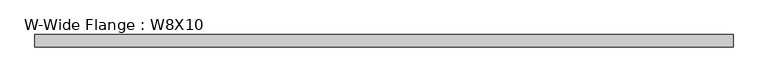
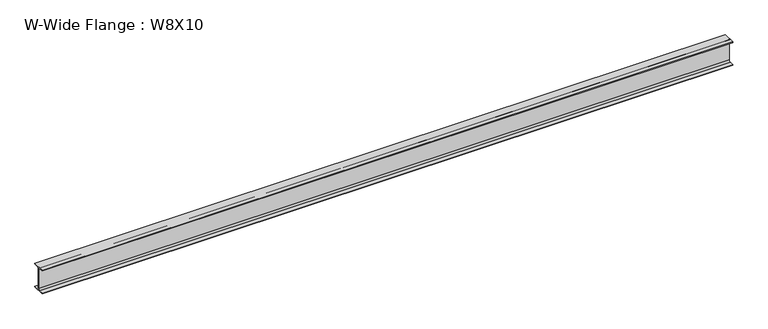
"""IFC4 building model written with IfcOpenShell, lengths in millimetres: beam geometry, W-Wide Flange : W8X10."""

from ifc_helpers import new_model, si_unit, point, frame, frame_2d, origin, place, context, project, spatial, polyline, circle_curve, trimmed, segment, composite_curve, outline, extrude, source, transform, mapped, element, save


def w_wide_flange_w8x10_6a41b71d(model_context):
    return source(origin(), model_context, "Body", "SweptSolid", [
        extrude(outline(composite_curve([segment(polyline([(50.038, -94.996), (50.038, -100.203), (-50.038, -100.203), (-50.038, -94.996), (-14.4145, -94.996)]), True, "CONTINUOUS"), segment(trimmed(circle_curve(frame_2d((-14.4145, -82.7405)), 12.2555), [point((-14.4145, -94.996))], [point((-2.159, -82.7405))], True, "CARTESIAN"), True, "CONTINUOUS"), segment(polyline([(-2.159, -82.7405), (-2.159, 82.7405)]), True, "CONTINUOUS"), segment(trimmed(circle_curve(frame_2d((-14.4145, 82.7405)), 12.2555), [point((-2.159, 82.7405))], [point((-14.4145, 94.996))], True, "CARTESIAN"), True, "CONTINUOUS"), segment(polyline([(-14.4145, 94.996), (-50.038, 94.996), (-50.038, 100.203), (50.038, 100.203), (50.038, 94.996), (14.4145, 94.996)]), True, "CONTINUOUS"), segment(trimmed(circle_curve(frame_2d((14.4145, 82.7405)), 12.2555), [point((14.4145, 94.996))], [point((2.159, 82.7405))], True, "CARTESIAN"), True, "CONTINUOUS"), segment(polyline([(2.159, 82.7405), (2.159, -82.7405)]), True, "CONTINUOUS"), segment(trimmed(circle_curve(frame_2d((14.4145, -82.7405)), 12.2555), [point((2.159, -82.7405))], [point((14.4145, -94.996))], True, "CARTESIAN"), True, "CONTINUOUS"), segment(polyline([(14.4145, -94.996), (50.038, -94.996)]), True, "CONTINUOUS")], self_intersect=False)), frame((-2744.7378906, 0.0, 0.0), z_axis=(1.0, 0.0, 0.0), x_axis=(0.0, 1.0, 0.0)), (0.0, 0.0, 1.0), 5603.8253906),
    ])


if __name__ == "__main__":
    model = new_model("IFC4")
    model_context = context("Model", 3, world=origin())
    ifc_project = project(units=[si_unit("LENGTHUNIT", "METRE", prefix="MILLI")], contexts=[model_context])
    site = spatial("IfcSite", under=ifc_project)
    building = spatial("IfcBuilding", under=site)
    placement = place(None, origin())
    w_wide_flange_w8x10_shape = w_wide_flange_w8x10_6a41b71d(model_context)
    element("IfcBeam", 1, ObjectType="W-Wide Flange : W8X10", at=placement, inside=building, context=model_context, shape_type="MappedRepresentation", body=[
        mapped(w_wide_flange_w8x10_shape, transform((0.0, 0.0, 0.0), x_axis=(1.0, 0.0, 0.0), y_axis=(0.0, 1.0, 0.0), z_axis=(0.0, 0.0, 1.0))),
    ])
    save(model, "model.ifc")

# Revit data of these elements
# Type "W-Wide Flange : W8X10"
#   Assembly Code = "B10"
#   W = 10
#   Length [instance default] = 1524 mm
#   bf = 100.076 mm
#   d = 200.406 mm
#   k = 17.463 mm
#   k2 = 12.255 mm
#   tf = 5.207 mm
#   tw = 4.318 mm
#   A = 0.00190967 m²
#   Structural Material [instance default] = Steel ASTM A992
# Element 1 (IfcBeam, "W-Wide Flange : W8X10")
#   Structural Material = Aluminum, Anodized Red
#   Materials on its faces: "Aluminum, Anodized Red"
# Materials
#   "Steel ASTM A992": class "Metal", colour RGB 128 0 0, transparency 0, Description = "Structural steel 50ksi", Cost = 0
#   "Aluminum, Anodized Red": class "Metal", colour RGB 120 120 120, transparency 0, Description = "Anodized aluminum, red", Cost = 0
